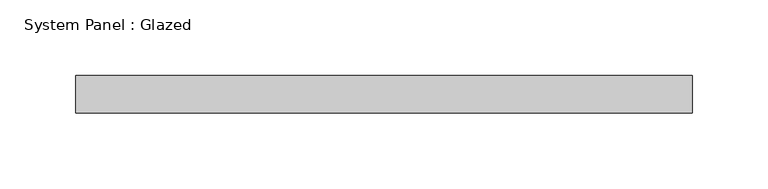
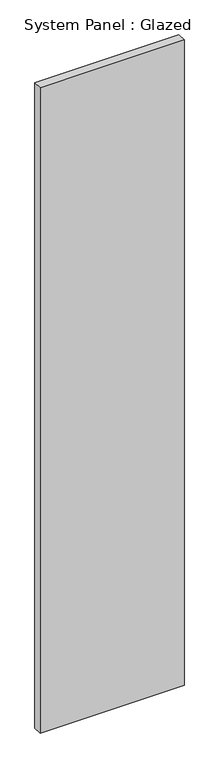
"""IFC4 building model written with IfcOpenShell, lengths in millimetres: plate geometry, System Panel : Glazed."""

from ifc_helpers import new_model, si_unit, origin, origin_with_axes, place, context, project, spatial, polyline, outline, extrude, source, transform, mapped, element, save


def system_panel_glazed_4745cc14(model_context):
    return source(origin(), model_context, "Body", "SweptSolid", [
        extrude(outline(polyline([(204.2039403, -49.5), (-204.2039403, -49.5), (-204.2039403, -24.5), (204.2039403, -24.5), (204.2039403, -49.5)])), origin_with_axes(), (0.0, 0.0, 1.0), 1934.1016494),
    ])


if __name__ == "__main__":
    model = new_model("IFC4")
    model_context = context("Model", 3, world=origin())
    ifc_project = project(units=[si_unit("LENGTHUNIT", "METRE", prefix="MILLI")], contexts=[model_context])
    site = spatial("IfcSite", under=ifc_project)
    building = spatial("IfcBuilding", under=site)
    placement = place(None, origin())
    system_panel_glazed_shape = system_panel_glazed_4745cc14(model_context)
    element("IfcPlate", 1, ObjectType="System Panel : Glazed", at=placement, inside=building, context=model_context, shape_type="MappedRepresentation", body=[
        mapped(system_panel_glazed_shape, transform((0.0, 0.0, 0.0), x_axis=(1.0, 0.0, 0.0), y_axis=(0.0, 1.0, 0.0), z_axis=(0.0, 0.0, 1.0))),
    ])
    save(model, "model.ifc")

# Revit data of these elements
# Type "System Panel : Glazed"
#   Keynote = "H11"
#   Construction Type Id = "GSP4R"
#   Analytic Construction = "1/8 in Pilkington single glazing"
#   Visual Light Transmittance = 0.9
#   Solar Heat Gain Coefficient = 0.86
#   Heat Transfer Coefficient (U) = 6.7069 W/(m²·K)
#   Define Thermal Properties by = 1
# Element 1 (IfcPlate, "System Panel : Glazed")
#   Materials on its faces: "Glass"
# Materials
#   "Glass": class "Glass", colour RGB 0 128 192, transparency 0.9, Description = "Soda Lime Glass", Cost = 0
